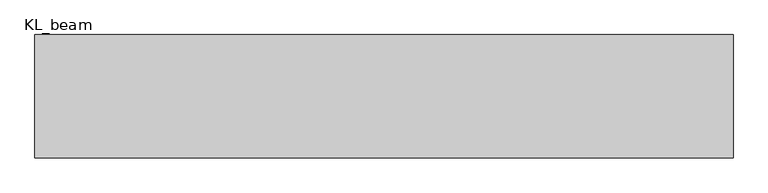
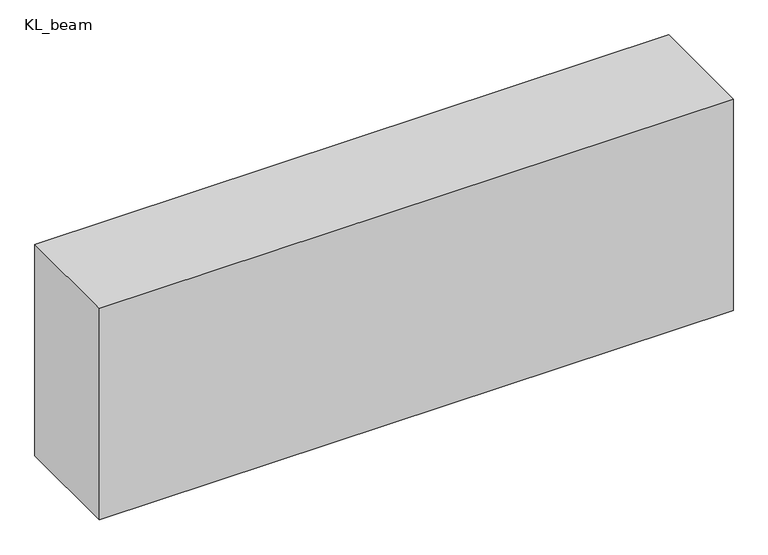
"""IFC4 building model written with IfcOpenShell, lengths in millimetres: beam geometry, 混凝土 - 矩形梁 : KL_beam."""

from ifc_helpers import new_model, si_unit, frame, origin, place, context, project, spatial, polyline, outline, extrude, source, transform, mapped, element, save


def kl_beam_2b0aae00(model_context):
    return source(origin(), model_context, "Body", "SweptSolid", [
        extrude(outline(polyline([(1133.5, 200.0), (1133.5, -200.0), (-1133.5, -200.0), (-1133.5, 200.0), (1133.5, 200.0)])), frame((0.0, 0.0, -400.0), z_axis=(0.0, 0.0, 1.0), x_axis=(1.0, 0.0, 0.0)), (0.0, 0.0, 1.0), 800.0),
    ])


if __name__ == "__main__":
    model = new_model("IFC4")
    model_context = context("Model", 3, world=origin())
    ifc_project = project(units=[si_unit("LENGTHUNIT", "METRE", prefix="MILLI")], contexts=[model_context])
    site = spatial("IfcSite", under=ifc_project)
    building = spatial("IfcBuilding", under=site)
    placement = place(None, origin())
    kl_beam_shape = kl_beam_2b0aae00(model_context)
    element("IfcBeam", 1, ObjectType="混凝土 - 矩形梁 : KL_beam", at=placement, inside=building, context=model_context, shape_type="MappedRepresentation", body=[
        mapped(kl_beam_shape, transform((0.0, 0.0, 0.0), x_axis=(1.0, 0.0, 0.0), y_axis=(0.0, 1.0, 0.0), z_axis=(0.0, 0.0, 1.0))),
    ])
    save(model, "model.ifc")

# Revit data of these elements
# Type "混凝土 - 矩形梁 : KL_beam"
#   Length [instance default] = 1524 mm
#   b = 400 mm
#   h = 800 mm
#   Structural Material [instance default] = 混凝土 - 现场浇注混凝土
#   Assembly Code = ""
# Element 1 (IfcBeam, "混凝土 - 矩形梁 : KL_beam")
#   Structural Material = none
# Materials
#   "混凝土 - 现场浇注混凝土": class "混凝土", colour RGB 192 192 192, transparency 0
